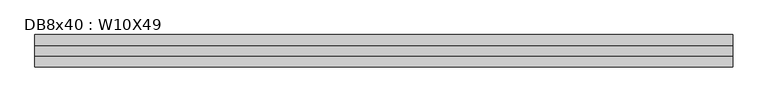
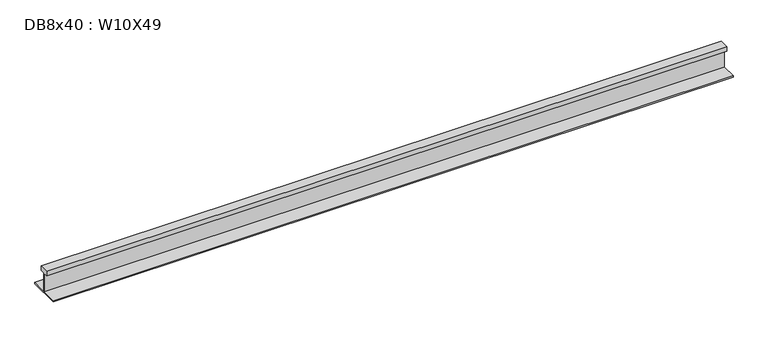
"""IFC4 building model written with IfcOpenShell, lengths in millimetres: beam geometry, DB8x40 : W10X49."""

from ifc_helpers import new_model, si_unit, frame, origin, place, context, project, spatial, polyline, outline, extrude, source, transform, mapped, element, save


def db8x40_w10x49_a1c94d84(model_context):
    return source(origin(), model_context, "Body", "SweptSolid", [
        extrude(outline(polyline([(38.1, 144.3355), (38.1, 106.2355), (2.921, 106.2355), (2.921, -49.53), (127.0, -49.53), (127.0, -59.182), (-127.0, -59.182), (-127.0, -49.53), (-2.921, -49.53), (-2.921, 106.2355), (-38.1, 106.2355), (-38.1, 144.3355), (38.1, 144.3355)])), frame((-2731.008, 0.0, 0.0), z_axis=(1.0, 0.0, 0.0), x_axis=(0.0, 1.0, 0.0)), (0.0, 0.0, 1.0), 5462.016),
    ])


if __name__ == "__main__":
    model = new_model("IFC4")
    model_context = context("Model", 3, world=origin())
    ifc_project = project(units=[si_unit("LENGTHUNIT", "METRE", prefix="MILLI")], contexts=[model_context])
    site = spatial("IfcSite", under=ifc_project)
    building = spatial("IfcBuilding", under=site)
    placement = place(None, origin())
    db8x40_w10x49_shape = db8x40_w10x49_a1c94d84(model_context)
    element("IfcBeam", 1, ObjectType="DB8x40 : W10X49", at=placement, inside=building, context=model_context, shape_type="MappedRepresentation", body=[
        mapped(db8x40_w10x49_shape, transform((0.0, 0.0, 0.0), x_axis=(1.0, 0.0, 0.0), y_axis=(0.0, 1.0, 0.0), z_axis=(0.0, 0.0, 1.0))),
    ])
    save(model, "model.ifc")

# Revit data of these elements
# Type "DB8x40 : W10X49"
#   Assembly Code = "B10"
#   W = 53
#   Length [instance default] = 5' - 0"
#   bf = 0' - 10"
#   d = 1' - 0.1"
#   k = 0' - 1 3/8"
#   k2 = 0' - 0.8"
#   tf = 0' - 0.575"
#   tw = 0' - 0.345"
#   A = 0.108333 SF
#   Structural Material [instance default] = Steel ASTM A992
# Element 1 (IfcBeam, "DB8x40 : W10X49")
#   Materials on its faces: "Steel ASTM A992"
# Materials
#   "Steel ASTM A992": class "Metal", colour RGB 199 199 199, transparency 0, Description = "Structural steel 50ksi", Cost = 0
